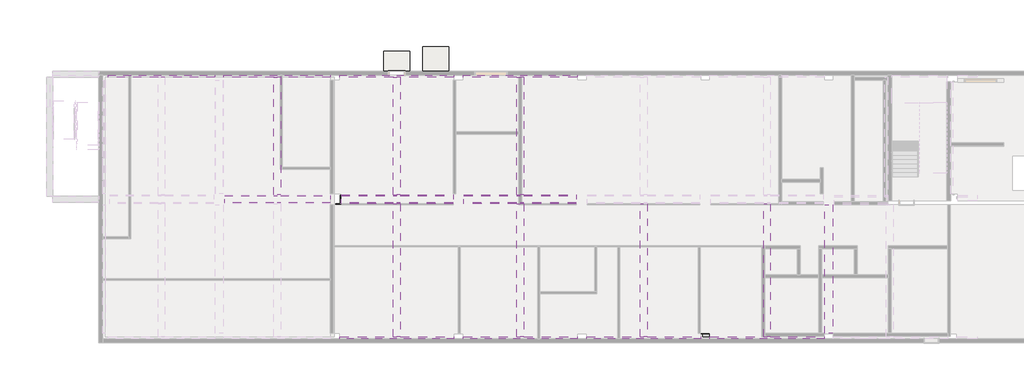
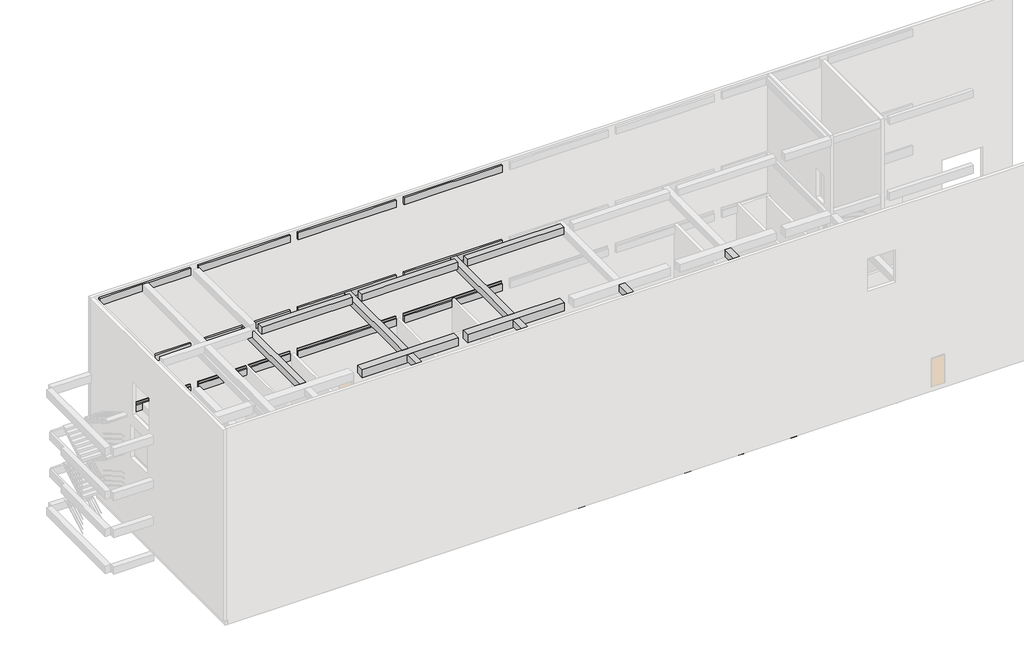
# One storey, part 3 of 5: 54 beams, 2 slabs.
# Revit data of these elements (continued)
# Type "RC Beam_Rectangular : H_SB_AR_S16_UG_B500xH700_1G1"
#   Type Comments = "CV-UG"
#   Type Mark = "1G1"
#   H_Q'ty Cal Type Tag = "SB-Q1"
#   H_WM Code_1 = "A03AF032-00022 |  | M3 | Concrete Work | Superstructure Work | Structural Concrete | Cement Type-1 | 25MPa ≤ F'c (Cylinder Strength) < 30MPa |  |  |  |  | A03AF032-00022 Concrete Work Superstructure Work Structural Concrete  Cement Type-1 25MPa ≤ F'c (Cylinder Strength) < 30MPa      |  F'c (Cylinder Strength) = 24MPa"
#   H_WM Code_2 = "A03AD037-00002 |  | TON | Concrete Work | Substructure Work | Rebar Work | Deformed Bar (Non-Coat.) | 400MPa<Fy≤470MPa |  |  |  |  | A03AD037-00002 Concrete Work Substructure Work Rebar Work Deformed Bar (Non-Coat.)  400MPa<Fy≤470MPa      | ASTM A615 GRADE 60 (Fy=420MPa)"
#   H_WM Code_3 = "A03AF036-00001 |  | M2 | Concrete Work | Superstructure Work | Form Work (1 time in use) | Flat Form | Dressed Lumber, Plywood or Steel Form(Wood Planks are not Allowed) incl. Chamfer |  |  |  | A03AF036-00001 Concrete Work Superstructure Work Form Work (1 time in use) Flat Form     Dressed Lumber, Plywood or Steel Form(Wood Planks are not Allowed) incl. Chamfer   |"
#   중앙부 하부근 = ""
#   중앙부 상부근 = ""
#   중앙부 보조근 = ""
#   중앙부 늑근 = ""
#   외단부 하부근 = ""
#   외단부 상부근 = ""
#   외단부 보조근 = ""
#   외단부 늑근 = ""
#   부호 = "TG2"
#   내단부 하부근 = ""
#   내단부 상부근 = ""
#   내단부 보조근 = ""
#   내단부 늑근 = ""
#   ALL 하부근 = "3-D20"
#   ALL 상부근 = "4-D20"
#   ALL 보조근 = ""
#   ALL 늑근 = "2-D10 @120"
#   H_Rebar ratio = 0.14
#   Width = 500 mm
#   Height = 700 mm
#   Length [instance default] = 1524 mm
#   b = 500 mm
#   h = 700 mm
#   hec_material3 [instance default] = none
#   hec_material2 [instance default] = none
#   hec_material1 [instance default] = none
#   Structural Material [instance default] = none
#   Assembly Code = ""
# Type "RC Beam_Rectangular : H_SB_AR_S16_UG_B450xH700_1B1A"
#   Type Comments = "UG"
#   Type Mark = "1B1A"
#   H_Q'ty Cal Type Tag = "SB-Q1"
#   H_WM Code_1 = "A03AF032-00022 |  | M3 | Concrete Work | Superstructure Work | Structural Concrete | Cement Type-1 | 25MPa ≤ F'c (Cylinder Strength) < 30MPa |  |  |  |  | A03AF032-00022 Concrete Work Superstructure Work Structural Concrete  Cement Type-1 25MPa ≤ F'c (Cylinder Strength) < 30MPa      |  F'c (Cylinder Strength) = 24MPa"
#   H_WM Code_2 = "A03AD037-00002 |  | TON | Concrete Work | Substructure Work | Rebar Work | Deformed Bar (Non-Coat.) | 400MPa<Fy≤470MPa |  |  |  |  | A03AD037-00002 Concrete Work Substructure Work Rebar Work Deformed Bar (Non-Coat.)  400MPa<Fy≤470MPa      | ASTM A615 GRADE 60 (Fy=420MPa)"
#   H_WM Code_3 = "A03AF036-00001 |  | M2 | Concrete Work | Superstructure Work | Form Work (1 time in use) | Flat Form | Dressed Lumber, Plywood or Steel Form(Wood Planks are not Allowed) incl. Chamfer |  |  |  | A03AF036-00001 Concrete Work Superstructure Work Form Work (1 time in use) Flat Form     Dressed Lumber, Plywood or Steel Form(Wood Planks are not Allowed) incl. Chamfer   |"
#   중앙부 하부근 = ""
#   중앙부 상부근 = ""
#   중앙부 보조근 = ""
#   중앙부 늑근 = ""
#   외단부 하부근 = ""
#   외단부 상부근 = ""
#   외단부 보조근 = ""
#   외단부 늑근 = ""
#   부호 = "TG2"
#   내단부 하부근 = ""
#   내단부 상부근 = ""
#   내단부 보조근 = ""
#   내단부 늑근 = ""
#   ALL 하부근 = "3-D20"
#   ALL 상부근 = "4-D20"
#   ALL 보조근 = ""
#   ALL 늑근 = "2-D10 @120"
#   Width = 450 mm
#   Height = 700 mm
#   Length [instance default] = 1524 mm
#   b = 450 mm
#   h = 700 mm
#   hec_material3 [instance default] = none
#   hec_material2 [instance default] = none
#   hec_material1 [instance default] = none
#   Structural Material [instance default] = none
#   Assembly Code = ""
# Type "RC Beam_Rectangular : H_SB_AR_S16_AG_B400xH700_3WG1"
#   Type Comments = "CV-AG"
#   Type Mark = "3WG1"
#   H_Q'ty Cal Type Tag = "SB-Q1"
#   H_WM Code_1 = "A03AF032-00022 |  | M3 | Concrete Work | Superstructure Work | Structural Concrete | Cement Type-1 | 25MPa ≤ F'c (Cylinder Strength) < 30MPa |  |  |  |  | A03AF032-00022 Concrete Work Superstructure Work Structural Concrete  Cement Type-1 25MPa ≤ F'c (Cylinder Strength) < 30MPa      |  F'c (Cylinder Strength) = 24MPa"
#   H_WM Code_2 = "A03AD037-00002 |  | TON | Concrete Work | Substructure Work | Rebar Work | Deformed Bar (Non-Coat.) | 400MPa<Fy≤470MPa |  |  |  |  | A03AD037-00002 Concrete Work Substructure Work Rebar Work Deformed Bar (Non-Coat.)  400MPa<Fy≤470MPa      | ASTM A615 GRADE 60 (Fy=420MPa)"
#   H_WM Code_3 = "A03AF036-00001 |  | M2 | Concrete Work | Superstructure Work | Form Work (1 time in use) | Flat Form | Dressed Lumber, Plywood or Steel Form(Wood Planks are not Allowed) incl. Chamfer |  |  |  | A03AF036-00001 Concrete Work Superstructure Work Form Work (1 time in use) Flat Form     Dressed Lumber, Plywood or Steel Form(Wood Planks are not Allowed) incl. Chamfer   |"
#   중앙부 하부근 = ""
#   중앙부 상부근 = ""
#   중앙부 보조근 = ""
#   중앙부 늑근 = ""
#   외단부 하부근 = ""
#   외단부 상부근 = ""
#   외단부 보조근 = ""
#   외단부 늑근 = ""
#   부호 = "TG2"
#   내단부 하부근 = ""
#   내단부 상부근 = ""
#   내단부 보조근 = ""
#   내단부 늑근 = ""
#   ALL 하부근 = "3-D20"
#   ALL 상부근 = "4-D20"
#   ALL 보조근 = ""
#   ALL 늑근 = "2-D10 @120"
#   H_Rebar ratio = 0.14
#   Width = 400 mm
#   Height = 700 mm
#   Length [instance default] = 1524 mm
#   b = 400 mm
#   h = 700 mm
#   hec_material3 [instance default] = none
#   hec_material2 [instance default] = none
#   hec_material1 [instance default] = none
#   Structural Material [instance default] = none
#   Assembly Code = ""
# Type "RC Beam_Rectangular : H_SB_AR_S16_AG_B600xH800_3G2"
#   Type Comments = "AG"
#   Type Mark = "3G2"
#   H_Q'ty Cal Type Tag = "SB-Q1"
#   H_WM Code_1 = "A03AF032-00022 |  | M3 | Concrete Work | Superstructure Work | Structural Concrete | Cement Type-1 | 25MPa ≤ F'c (Cylinder Strength) < 30MPa |  |  |  |  | A03AF032-00022 Concrete Work Superstructure Work Structural Concrete  Cement Type-1 25MPa ≤ F'c (Cylinder Strength) < 30MPa      |  F'c (Cylinder Strength) = 24MPa"
#   H_WM Code_2 = "A03AD037-00002 |  | TON | Concrete Work | Substructure Work | Rebar Work | Deformed Bar (Non-Coat.) | 400MPa<Fy≤470MPa |  |  |  |  | A03AD037-00002 Concrete Work Substructure Work Rebar Work Deformed Bar (Non-Coat.)  400MPa<Fy≤470MPa      | ASTM A615 GRADE 60 (Fy=420MPa)"
#   H_WM Code_3 = "A03AF036-00001 |  | M2 | Concrete Work | Superstructure Work | Form Work (1 time in use) | Flat Form | Dressed Lumber, Plywood or Steel Form(Wood Planks are not Allowed) incl. Chamfer |  |  |  | A03AF036-00001 Concrete Work Superstructure Work Form Work (1 time in use) Flat Form     Dressed Lumber, Plywood or Steel Form(Wood Planks are not Allowed) incl. Chamfer   |"
#   중앙부 하부근 = ""
#   중앙부 상부근 = ""
#   중앙부 보조근 = ""
#   중앙부 늑근 = ""
#   외단부 하부근 = ""
#   외단부 상부근 = ""
#   외단부 보조근 = ""
#   외단부 늑근 = ""
#   부호 = "TG2"
#   내단부 하부근 = ""
#   내단부 상부근 = ""
#   내단부 보조근 = ""
#   내단부 늑근 = ""
#   ALL 하부근 = "3-D20"
#   ALL 상부근 = "4-D20"
#   ALL 보조근 = ""
#   ALL 늑근 = "2-D10 @120"
#   Width = 600 mm
#   Height = 800 mm
#   Length [instance default] = 1524 mm
#   b = 600 mm
#   h = 800 mm
#   hec_material3 [instance default] = none
#   hec_material2 [instance default] = none
#   hec_material1 [instance default] = none
#   Structural Material [instance default] = none
#   Assembly Code = ""
# Type "RC Beam_Rectangular : H_SB_AR_S16_AG_B4500xH700_3G1"
#   Type Comments = "AG"
#   Type Mark = "3G1"
#   H_Q'ty Cal Type Tag = "SB-Q1"
#   H_WM Code_1 = "A03AF032-00022 |  | M3 | Concrete Work | Superstructure Work | Structural Concrete | Cement Type-1 | 25MPa ≤ F'c (Cylinder Strength) < 30MPa |  |  |  |  | A03AF032-00022 Concrete Work Superstructure Work Structural Concrete  Cement Type-1 25MPa ≤ F'c (Cylinder Strength) < 30MPa      |  F'c (Cylinder Strength) = 24MPa"
#   H_WM Code_2 = "A03AD037-00002 |  | TON | Concrete Work | Substructure Work | Rebar Work | Deformed Bar (Non-Coat.) | 400MPa<Fy≤470MPa |  |  |  |  | A03AD037-00002 Concrete Work Substructure Work Rebar Work Deformed Bar (Non-Coat.)  400MPa<Fy≤470MPa      | ASTM A615 GRADE 60 (Fy=420MPa)"
#   H_WM Code_3 = "A03AF036-00001 |  | M2 | Concrete Work | Superstructure Work | Form Work (1 time in use) | Flat Form | Dressed Lumber, Plywood or Steel Form(Wood Planks are not Allowed) incl. Chamfer |  |  |  | A03AF036-00001 Concrete Work Superstructure Work Form Work (1 time in use) Flat Form     Dressed Lumber, Plywood or Steel Form(Wood Planks are not Allowed) incl. Chamfer   |"
#   중앙부 하부근 = ""
#   중앙부 상부근 = ""
#   중앙부 보조근 = ""
#   중앙부 늑근 = ""
#   외단부 하부근 = ""
#   외단부 상부근 = ""
#   외단부 보조근 = ""
#   외단부 늑근 = ""
#   부호 = "TG2"
#   내단부 하부근 = ""
#   내단부 상부근 = ""
#   내단부 보조근 = ""
#   내단부 늑근 = ""
#   ALL 하부근 = "3-D20"
#   ALL 상부근 = "4-D20"
#   ALL 보조근 = ""
#   ALL 늑근 = "2-D10 @120"
#   Width = 500 mm
#   Height = 700 mm
#   Length [instance default] = 1524 mm
#   b = 500 mm
#   h = 700 mm
#   hec_material3 [instance default] = none
#   hec_material2 [instance default] = none
#   hec_material1 [instance default] = none
#   Structural Material [instance default] = none
#   Assembly Code = ""
# Type "RC Beam_Rectangular : H_SB_AR_S16_AG_B450xH700_3B1"
#   Type Comments = "AG"
#   Type Mark = "3B1"
#   H_Q'ty Cal Type Tag = "SB-Q1"
#   H_WM Code_1 = "A03AF032-00022 |  | M3 | Concrete Work | Superstructure Work | Structural Concrete | Cement Type-1 | 25MPa ≤ F'c (Cylinder Strength) < 30MPa |  |  |  |  | A03AF032-00022 Concrete Work Superstructure Work Structural Concrete  Cement Type-1 25MPa ≤ F'c (Cylinder Strength) < 30MPa      |  F'c (Cylinder Strength) = 24MPa"
#   H_WM Code_2 = "A03AD037-00002 |  | TON | Concrete Work | Substructure Work | Rebar Work | Deformed Bar (Non-Coat.) | 400MPa<Fy≤470MPa |  |  |  |  | A03AD037-00002 Concrete Work Substructure Work Rebar Work Deformed Bar (Non-Coat.)  400MPa<Fy≤470MPa      | ASTM A615 GRADE 60 (Fy=420MPa)"
#   H_WM Code_3 = "A03AF036-00001 |  | M2 | Concrete Work | Superstructure Work | Form Work (1 time in use) | Flat Form | Dressed Lumber, Plywood or Steel Form(Wood Planks are not Allowed) incl. Chamfer |  |  |  | A03AF036-00001 Concrete Work Superstructure Work Form Work (1 time in use) Flat Form     Dressed Lumber, Plywood or Steel Form(Wood Planks are not Allowed) incl. Chamfer   |"
#   중앙부 하부근 = ""
#   중앙부 상부근 = ""
#   중앙부 보조근 = ""
#   중앙부 늑근 = ""
#   외단부 하부근 = ""
#   외단부 상부근 = ""
#   외단부 보조근 = ""
#   외단부 늑근 = ""
#   부호 = "TG2"
#   내단부 하부근 = ""
#   내단부 상부근 = ""
#   내단부 보조근 = ""
#   내단부 늑근 = ""
#   ALL 하부근 = "3-D20"
#   ALL 상부근 = "4-D20"
#   ALL 보조근 = ""
#   ALL 늑근 = "2-D10 @120"
#   Width = 450 mm
#   Height = 700 mm
#   Length [instance default] = 1524 mm
#   b = 450 mm
#   h = 700 mm
#   hec_material3 [instance default] = none
#   hec_material2 [instance default] = none
#   hec_material1 [instance default] = none
#   Structural Material [instance default] = none
#   Assembly Code = ""
# Type "RC Beam_Rectangular : H_SB_AR_S16_AG_B450xH700_3B1A"
#   Type Comments = "AG"
#   Type Mark = "3B1A"
#   H_Q'ty Cal Type Tag = "SB-Q1"
#   H_WM Code_1 = "A03AF032-00022 |  | M3 | Concrete Work | Superstructure Work | Structural Concrete | Cement Type-1 | 25MPa ≤ F'c (Cylinder Strength) < 30MPa |  |  |  |  | A03AF032-00022 Concrete Work Superstructure Work Structural Concrete  Cement Type-1 25MPa ≤ F'c (Cylinder Strength) < 30MPa      |  F'c (Cylinder Strength) = 24MPa"
#   H_WM Code_2 = "A03AD037-00002 |  | TON | Concrete Work | Substructure Work | Rebar Work | Deformed Bar (Non-Coat.) | 400MPa<Fy≤470MPa |  |  |  |  | A03AD037-00002 Concrete Work Substructure Work Rebar Work Deformed Bar (Non-Coat.)  400MPa<Fy≤470MPa      | ASTM A615 GRADE 60 (Fy=420MPa)"
#   H_WM Code_3 = "A03AF036-00001 |  | M2 | Concrete Work | Superstructure Work | Form Work (1 time in use) | Flat Form | Dressed Lumber, Plywood or Steel Form(Wood Planks are not Allowed) incl. Chamfer |  |  |  | A03AF036-00001 Concrete Work Superstructure Work Form Work (1 time in use) Flat Form     Dressed Lumber, Plywood or Steel Form(Wood Planks are not Allowed) incl. Chamfer   |"
#   중앙부 하부근 = ""
#   중앙부 상부근 = ""
#   중앙부 보조근 = ""
#   중앙부 늑근 = ""
#   외단부 하부근 = ""
#   외단부 상부근 = ""
#   외단부 보조근 = ""
#   외단부 늑근 = ""
#   부호 = "TG2"
#   내단부 하부근 = ""
#   내단부 상부근 = ""
#   내단부 보조근 = ""
#   내단부 늑근 = ""
#   ALL 하부근 = "3-D20"
#   ALL 상부근 = "4-D20"
#   ALL 보조근 = ""
#   ALL 늑근 = "2-D10 @120"
#   Width = 450 mm
#   Height = 700 mm
#   Length [instance default] = 1524 mm
#   b = 450 mm
#   h = 700 mm
#   hec_material3 [instance default] = none
#   hec_material2 [instance default] = none
#   hec_material1 [instance default] = none
#   Structural Material [instance default] = none
#   Assembly Code = ""
# Type "RC Beam_Rectangular : H_SB_AR_S16_AG_B400xH700_RWG1"
#   Type Comments = "CV-AG"
#   Type Mark = "RWG1"
#   H_Q'ty Cal Type Tag = "SB-Q1"
#   H_WM Code_1 = "A03AF032-00022 |  | M3 | Concrete Work | Superstructure Work | Structural Concrete | Cement Type-1 | 25MPa ≤ F'c (Cylinder Strength) < 30MPa |  |  |  |  | A03AF032-00022 Concrete Work Superstructure Work Structural Concrete  Cement Type-1 25MPa ≤ F'c (Cylinder Strength) < 30MPa      |  F'c (Cylinder Strength) = 24MPa"
#   H_WM Code_2 = "A03AD037-00002 |  | TON | Concrete Work | Substructure Work | Rebar Work | Deformed Bar (Non-Coat.) | 400MPa<Fy≤470MPa |  |  |  |  | A03AD037-00002 Concrete Work Substructure Work Rebar Work Deformed Bar (Non-Coat.)  400MPa<Fy≤470MPa      | ASTM A615 GRADE 60 (Fy=420MPa)"
#   H_WM Code_3 = "A03AF036-00001 |  | M2 | Concrete Work | Superstructure Work | Form Work (1 time in use) | Flat Form | Dressed Lumber, Plywood or Steel Form(Wood Planks are not Allowed) incl. Chamfer |  |  |  | A03AF036-00001 Concrete Work Superstructure Work Form Work (1 time in use) Flat Form     Dressed Lumber, Plywood or Steel Form(Wood Planks are not Allowed) incl. Chamfer   |"
#   중앙부 하부근 = ""
#   중앙부 상부근 = ""
#   중앙부 보조근 = ""
#   중앙부 늑근 = ""
#   외단부 하부근 = ""
#   외단부 상부근 = ""
#   외단부 보조근 = ""
#   외단부 늑근 = ""
#   부호 = "TG2"
#   내단부 하부근 = ""
#   내단부 상부근 = ""
#   내단부 보조근 = ""
#   내단부 늑근 = ""
#   ALL 하부근 = "3-D20"
#   ALL 상부근 = "4-D20"
#   ALL 보조근 = ""
#   ALL 늑근 = "2-D10 @120"
#   H_Rebar ratio = 0.14
#   Width = 400 mm
#   Height = 700 mm
#   Length [instance default] = 1524 mm
#   b = 400 mm
#   h = 700 mm
#   hec_material3 [instance default] = none
#   hec_material2 [instance default] = none
#   hec_material1 [instance default] = none
#   Structural Material [instance default] = none
#   Assembly Code = ""
# Type "RC Beam_Rectangular : H_SB_AR_S16_AG_B450xH700_RG2"
#   Type Comments = "AG"
#   Type Mark = "RG2"
#   H_Q'ty Cal Type Tag = "SB-Q1"
#   H_WM Code_1 = "A03AF032-00022 |  | M3 | Concrete Work | Superstructure Work | Structural Concrete | Cement Type-1 | 25MPa ≤ F'c (Cylinder Strength) < 30MPa |  |  |  |  | A03AF032-00022 Concrete Work Superstructure Work Structural Concrete  Cement Type-1 25MPa ≤ F'c (Cylinder Strength) < 30MPa      |  F'c (Cylinder Strength) = 24MPa"
#   H_WM Code_2 = "A03AD037-00002 |  | TON | Concrete Work | Substructure Work | Rebar Work | Deformed Bar (Non-Coat.) | 400MPa<Fy≤470MPa |  |  |  |  | A03AD037-00002 Concrete Work Substructure Work Rebar Work Deformed Bar (Non-Coat.)  400MPa<Fy≤470MPa      | ASTM A615 GRADE 60 (Fy=420MPa)"
#   H_WM Code_3 = "A03AF036-00001 |  | M2 | Concrete Work | Superstructure Work | Form Work (1 time in use) | Flat Form | Dressed Lumber, Plywood or Steel Form(Wood Planks are not Allowed) incl. Chamfer |  |  |  | A03AF036-00001 Concrete Work Superstructure Work Form Work (1 time in use) Flat Form     Dressed Lumber, Plywood or Steel Form(Wood Planks are not Allowed) incl. Chamfer   |"
#   중앙부 하부근 = ""
#   중앙부 상부근 = ""
#   중앙부 보조근 = ""
#   중앙부 늑근 = ""
#   외단부 하부근 = ""
#   외단부 상부근 = ""
#   외단부 보조근 = ""
#   외단부 늑근 = ""
#   부호 = "TG2"
#   내단부 하부근 = ""
#   내단부 상부근 = ""
#   내단부 보조근 = ""
#   내단부 늑근 = ""
#   ALL 하부근 = "3-D20"
#   ALL 상부근 = "4-D20"
#   ALL 보조근 = ""
#   ALL 늑근 = "2-D10 @120"
#   Width = 450 mm
#   Height = 700 mm
#   Length [instance default] = 1524 mm
#   b = 450 mm
#   h = 700 mm
#   hec_material3 [instance default] = none
#   hec_material2 [instance default] = none
#   hec_material1 [instance default] = none
#   Structural Material [instance default] = none
#   Assembly Code = ""
# Type "H_SF_AR_B08_Ramp_Ramp2"
#   Type Comments = "CV-AG"
#   Type Mark = "Ramp2"
#   H_Q'ty Cal Type Tag = "SB-Q1A"
#   H_WM Code_1 = "A03AF032-00022 |  | M3 | Concrete Work | Superstructure Work | Structural Concrete | Cement Type-1 | 25MPa ≤ F'c (Cylinder Strength) < 30MPa |  |  |  |  | A03AF032-00022 Concrete Work Superstructure Work Structural Concrete  Cement Type-1 25MPa ≤ F'c (Cylinder Strength) < 30MPa      |  F'c (Cylinder Strength) = 24MPa"
#   H_WM Code_2 = "A03AD037-00002 |  | TON | Concrete Work | Substructure Work | Rebar Work | Deformed Bar (Non-Coat.) | 400MPa<Fy≤470MPa |  |  |  |  | A03AD037-00002 Concrete Work Substructure Work Rebar Work Deformed Bar (Non-Coat.)  400MPa<Fy≤470MPa      | ASTM A615 GRADE 60 (Fy=420MPa)"
#   H_WM Code_3 = "A03AD035-00001 |  | M2 | Concrete Work | Substructure Work | Form Work (3 times in use) | Flat Form | Dressed Lumber, Plywood or Steel Form(Wood Planks are not Allowed) incl. Chamfer |  |  |  | A03AD035-00001 Concrete Work Substructure Work Form Work (3 times in use) Flat Form     Dressed Lumber, Plywood or Steel Form(Wood Planks are not Allowed) incl. Chamfer   | Dressed Lumber, Plywood or Steel Form(Wood Planks are not Allowed) incl. Chamfer"
#   H_WM Code_4 = "A03AH056-00001 |  | M2 | Concrete Work | Concrete Protective Coating (U/G) | Bitumen/Bituminous/Asphalt Coating |  |  | A03AH056-00001 Concrete Work Concrete Protective Coating (U/G) Bitumen/Bituminous/Asphalt Coating         | Bitumen/Bituminous/Asphalt Coating"
#   H_WM Code_5 = "A03AD047-00004 |  | M2 | Concrete Work | Substructure Work | Insulation under Ground Floor | Extruded Polystyrene Insulation Board |  | 100mm≤THK | THK=(  )mm |  | A03AD047-00004 Concrete Work Substructure Work Insulation under Ground Floor Extruded Polystyrene Insulation Board       100mm≤THK | Bitumen/Bituminous/Asphalt Coating"
#   H_WM Code_6 = "A01ZZ001-00012 |  | M3 | Earth Work | - | Excavation | Soil, Mech. |  | Manual Excavation Above GWL |  |  |  | A01ZZ001-00012 Earth Work - Excavation Soil, Mech.      Manual Excavation Above GWL  | Above GWL"
#   H_WM Code_7 = "A01ZZ001-00013 |  | M3 | Earth Work | - | Excavation | Soil, Mech. |  | Manual Excavation Below GWL |  |  |  | A01ZZ001-00013 Earth Work - Excavation Soil, Mech.      Manual Excavation Below GWL  | Below GWL"
#   H_WM Code_8 = "A01ZZ003-00001 |  | M3 | Earth Work | - | Backfill | Re-use, Soil |  |  |  | Compaction=(  )% |  | A01ZZ003-00001 Earth Work - Backfill Re-use, Soil        | Compaction=( 95 )%"
#   H_WM Code_9 = "A01ZZ004-00001 |  | M3 | Earth Work | - | Disposal | Soil |  |  |  | Disposal Distance=Appx. (  )km from Site |  | A01ZZ004-00001 Earth Work - Disposal Soil        | Disposal Distance=Appx. (20 )km from Site"
#   H_WM Code_10 = "A03AH056-00001 |  | M2 | Concrete Work | Concrete Protective Coating (U/G) | Bitumen/Bituminous/Asphalt Coating |  |  | A03AH056-00001 Concrete Work Concrete Protective Coating (U/G) Bitumen/Bituminous/Asphalt Coating         | *기초바닥 Protection 은 Lean에 적용"
#   H_Rebar ratio = 0.1
#   Layers, outside or top first: 0 mm no material (function 100); 200 mm "00_Concrete_Reinf. Conc." (function 1); 0 mm no material (function 100); 0 mm no material (function 100)
# Element 1 (IfcBeam, "RC Beam_Rectangular : H_SB_AR_S16_UG_B600xH800_1G2")
#   Comments = ""
#   hec_material3 = none
#   hec_material2 = none
#   hec_material1 = none
#   Structural Material = 00_Concrete_Reinf. Conc.
#   Phase Created = New Construction
#   Materials on its faces: "00_Concrete_Reinf. Conc."
# Elements 2, 3 (IfcBeam, "RC Beam_Rectangular : H_SB_AR_S16_UG_B450xH700_1B1")
#   Comments = ""
#   hec_material3 = none
#   hec_material2 = none
#   hec_material1 = none
#   Structural Material = 00_Concrete_Reinf. Conc.
#   Phase Created = New Construction
#   Materials on its faces: "00_Concrete_Reinf. Conc."
# Elements 4, 5, 6, 7, 8, 9 (IfcBeam, "RC Beam_Rectangular : H_SB_AR_S16_UG_B500xH700_1G1")
#   Comments = ""
#   hec_material3 = none
#   hec_material2 = none
#   hec_material1 = none
#   Structural Material = 00_Concrete_Reinf. Conc.
#   Phase Created = New Construction
#   Materials on its faces: "00_Concrete_Reinf. Conc."
# Elements 10, 11, 12, 13 (IfcBeam, "RC Beam_Rectangular : H_SB_AR_S16_UG_B450xH700_1B1A")
#   Comments = ""
#   hec_material3 = none
#   hec_material2 = none
#   hec_material1 = none
#   Structural Material = none
#   Phase Created = New Construction
# Elements 14, 15, 16, 17, 18, 19, 20, 21, 25, 26, 27, 28, 29, 30, 31, 32 (IfcBeam, "RC Beam_Rectangular : H_SB_AR_S16_AG_B400xH700_3WG1")
#   Comments = ""
#   hec_material3 = none
#   hec_material2 = none
#   hec_material1 = none
#   Structural Material = 00_Concrete_Reinf. Conc.
#   Phase Created = New Construction
#   Materials on its faces: "00_Concrete_Reinf. Conc."
# Elements 22, 23, 33, 34 (IfcBeam, "RC Beam_Rectangular : H_SB_AR_S16_AG_B600xH800_3G2")
#   Comments = ""
#   hec_material3 = none
#   hec_material2 = none
#   hec_material1 = none
#   Structural Material = none
#   Phase Created = New Construction
# Element 24 (IfcBeam, "RC Beam_Rectangular : H_SB_AR_S16_AG_B4500xH700_3G1")
#   Comments = ""
#   hec_material3 = none
#   hec_material2 = none
#   hec_material1 = none
#   Structural Material = none
#   Phase Created = New Construction
# Elements 35, 36, 37 (IfcBeam, "RC Beam_Rectangular : H_SB_AR_S16_AG_B450xH700_3B1")
#   Comments = ""
#   hec_material3 = none
#   hec_material2 = none
#   hec_material1 = none
#   Structural Material = none
#   Phase Created = New Construction
# Elements 38, 39, 40, 41 (IfcBeam, "RC Beam_Rectangular : H_SB_AR_S16_AG_B450xH700_3B1A")
#   Comments = ""
#   hec_material3 = none
#   hec_material2 = none
#   hec_material1 = none
#   Structural Material = none
#   Phase Created = New Construction
# Elements 42, 43, 44, 45, 46, 47, 48, 49 (IfcBeam, "RC Beam_Rectangular : H_SB_AR_S16_AG_B400xH700_RWG1")
#   Comments = ""
#   hec_material3 = none
#   hec_material2 = none
#   hec_material1 = none
#   Structural Material = 00_Concrete_Reinf. Conc.
#   Phase Created = New Construction
#   Materials on its faces: "00_Concrete_Reinf. Conc."
# Elements 50, 51, 52 (IfcBeam, "RC Beam_Rectangular : H_SB_AR_S16_AG_B450xH700_RG2")
#   Comments = ""
#   hec_material3 = none
#   hec_material2 = none
#   hec_material1 = none
#   Structural Material = none
#   Phase Created = New Construction
# Element 53 (IfcBeam, "RC Beam_Rectangular : H_SB_AR_S16_UG_B600xH800_1G2")
#   IfcGUID = "0DKOmQSjf1KgvfYSs63FG0"
#   Comments = ""
#   Phase Created = New Construction
#   Materials on its faces: "00_Concrete_Reinf. Conc."
# Element 54 (IfcBeam, "RC Beam_Rectangular : H_SB_AR_S16_UG_B600xH800_1G2")
#   IfcGUID = "0DKOmQSjf1KgvfYSs63FHI"
#   Comments = ""
#   Phase Created = New Construction
#   Materials on its faces: "00_Concrete_Reinf. Conc."
# Elements 55, 56 (IfcSlab, "H_SF_AR_B08_Ramp_Ramp2")
#   Comments = ""
#   built-in parameter 1001955 = 3.14159 (stored number, unit not read)
#   Height Offset From Level = 0 mm
#   built-in parameter 1001954 = 1
#   Phase Created = New Construction
# Materials
#   "00_Concrete_Reinf. Conc.": class "Concrete", colour RGB 176 176 176, transparency 0, Description = "Reinf. Conc.", Cost = 0, Image = Concrete.Cast-In-Place.Flat.Polished.Grey.jpg
# Room at (48881.519, 2598.242) mm, phase "New Construction", upper level "TOC", upper offset 9000 mm, lower offset 0 mm
#   Comments = ""
#   Number = "121"
#   Name = "TOILET (M)"
#   H_Floor Finish Style Name = "Non-Slip Unglazed Ceramic Tile"
#   H_Floor Base Material = "Concrete Slab / Screed / Liquid Waterproofing"
#   H_Wall-Base Material-1 = "Masonry Wall"
#   H_Wall-Base Material-2 = ""
#   H_Wall-Base Material-3 = ""
#   H_Floor-Base Material-1 = "Concrete Slab"
#   H_Floor-Base Material-2 = ""
#   H_Floor-Base Material-3 = "Screed"
#   H_Floor-Base Material-4 = "Liquid Waterproofing"
#   H_Floor-Base Material-5 = "Ceramic Tile"
#   H_Floor Finish-1 = "Ceramic Tile"
#   H_Floor Finish-2 = ""
#   H_Floor Finish Remark = ""
#   H_Wall Finish Style Name = "Glazed Ceramic Tile (≤C.H+100) / No Paint (>C.H+100)"
#   H_Wall Base Material = "Masonry Wall"
#   H_Wall-Base Material-4 = "No Waterproofing"
#   H_Wall-Base Material-5 = "Glazed Ceramic Tile"
#   H_Wall Finish-1 = "Glazed Ceramic Tile"
#   H_Wall Finish-2 = ""
#   H_Wall Finish Remark = "Below Suspended Ceiling\nGlazed Ceramic Tile(≤C.H+100) / No Paint (>C.H+100)"
#   H_Ceiling Finish Style Name = "Suspended Gypsum Plaster Board Ceiling (M-Bar)"
#   H_Ceiling Base Material = "Concrete Slab / Fair Faced Concrete"
#   H_Ceiling-Base Material-1 = "(Concrete Slab)"
#   H_Ceiling-Base Material-2 = "(Fair Faced Concrete)"
#   H_Ceiling-Base Material-3 = ""
#   H_Ceiling-Base Material-4 = ""
#   H_Ceiling-Base Material-5 = "Gypsum Plaster Board Ceiling System"
#   H_Ceiling Finish-1 = "Gypsum Plaster Board Ceiling System"
#   H_Ceiling Finish-2 = ""
#   H_Ceiling Finish Remark = ""
#   H_Room W = 3800 mm
#   H_Room L = 5600 mm
#   H_Room H or CH = 9000 mm
#   Floor Finish Style No = none
#   Wall Finish Style No = W32D
#   Ceiling Finish Style No = C92
# Room at (40583.851, 3309.471) mm, phase "New Construction", upper level "TOC", upper offset 9000 mm, lower offset 0 mm
#   Comments = ""
#   Number = "117"
#   Name = "PARTNER'S ROOM"
#   H_Floor Finish Style Name = "Vinyl Tile"
#   H_Floor Base Material = "Concrete Slab / Steel Trowel Finish"
#   H_Wall-Base Material-1 = "Masonry Wall"
#   H_Skirt Finish Style Name = "Coved Vinyl Tile"
#   H_Wall-Base Material-2 = ""
#   H_Wall-Base Material-3 = "Plastering"
#   H_Floor-Base Material-1 = "Concrete Slab"
#   H_Floor-Base Material-2 = "Steel Trowel Finish"
#   H_Floor-Base Material-3 = ""
#   H_Floor-Base Material-4 = ""
#   H_Floor-Base Material-5 = "Vinyl Tile"
#   H_Floor Finish-1 = "Vinyl Tile"
#   H_Floor Finish-2 = ""
#   H_Floor Finish Remark = ""
#   H_Skirt Base Material = "Same as Wall"
#   H_Skirt-Base Material-1 = ""
#   H_Skirt-Base Material-2 = ""
#   H_Skirt-Base Material-3 = ""
#   H_Skirt-Base Material-4 = ""
#   H_Skirt-Base Material-5 = ""
#   H_Skirt Finish-1 = "Vinyl Tile"
#   H_Skirt Finish-2 = ""
#   H_Skirt Finish Remark = "Vinyl Tile = PVC Tile (polyvinyl chloride)"
#   H_Wall Finish Style Name = "Water Emulsion Paint"
#   H_Wall Base Material = "Masonry Wall / Cement Plaster"
#   H_Wall-Base Material-4 = ""
#   H_Wall-Base Material-5 = ""
#   H_Wall Finish-1 = ""
#   H_Wall Finish-2 = ""
#   H_Wall Finish Remark = ""
#   H_Ceiling Finish Style Name = "Suspended Acoustic Tiled Ceiling (M-Bar)"
#   H_Ceiling Base Material = "Concrete Slab / Fair Faced Concrete"
#   H_Ceiling-Base Material-1 = "(Concrete Slab)"
#   H_Ceiling-Base Material-2 = "(Fair Faced Concrete)"
#   H_Ceiling-Base Material-3 = ""
#   H_Ceiling-Base Material-4 = ""
#   H_Ceiling-Base Material-5 = "Acoustic Tiled Ceiling System (M-Bar)"
#   H_Ceiling Finish-1 = "Acoustic Tiled Ceiling System (M-Bar)"
#   H_Ceiling Finish-2 = ""
#   H_Ceiling Finish Remark = ""
#   H_Room W = 3700 mm
#   H_Room L = 3700 mm
#   H_Room H or CH = 9000 mm
#   Floor Finish Style No = none
#   Skirt Finish Style No = none
#   Wall Finish Style No = W02B
#   Ceiling Finish Style No = C95A
# Room at (25580.312, 3648.151) mm, phase "New Construction", upper level "TOC", upper offset 9000 mm, lower offset 0 mm
#   Comments = ""
#   Number = "115"
#   Name = "REST ROOM"
#   H_Floor Finish Style Name = "Vinyl Tile"
#   H_Floor Base Material = "Concrete Slab / Steel Trowel Finish"
#   H_Wall-Base Material-1 = "Masonry Wall"
#   H_Skirt Finish Style Name = "Coved Vinyl Tile"
#   H_Wall-Base Material-2 = ""
#   H_Wall-Base Material-3 = "Plastering"
#   H_Floor-Base Material-1 = "Concrete Slab"
#   H_Floor-Base Material-2 = "Steel Trowel Finish"
#   H_Floor-Base Material-3 = ""
#   H_Floor-Base Material-4 = ""
#   H_Floor-Base Material-5 = "Vinyl Tile"
#   H_Floor Finish-1 = "Vinyl Tile"
#   H_Floor Finish-2 = ""
#   H_Floor Finish Remark = ""
#   H_Skirt Base Material = "Same as Wall"
#   H_Skirt-Base Material-1 = ""
#   H_Skirt-Base Material-2 = ""
#   H_Skirt-Base Material-3 = ""
#   H_Skirt-Base Material-4 = ""
#   H_Skirt-Base Material-5 = ""
#   H_Skirt Finish-1 = "Vinyl Tile"
#   H_Skirt Finish-2 = ""
#   H_Skirt Finish Remark = "Vinyl Tile = PVC Tile (polyvinyl chloride)"
#   H_Wall Finish Style Name = "Water Emulsion Paint"
#   H_Wall Base Material = "Masonry Wall / Cement Plaster"
#   H_Wall-Base Material-4 = ""
#   H_Wall-Base Material-5 = ""
#   H_Wall Finish-1 = ""
#   H_Wall Finish-2 = ""
#   H_Wall Finish Remark = ""
#   H_Ceiling Finish Style Name = "Suspended Gypsum Plaster Board Ceiling (M-Bar)"
#   H_Ceiling Base Material = "Concrete Slab / Fair Faced Concrete"
#   H_Ceiling-Base Material-1 = "(Concrete Slab)"
#   H_Ceiling-Base Material-2 = "(Fair Faced Concrete)"
#   H_Ceiling-Base Material-3 = ""
#   H_Ceiling-Base Material-4 = ""
#   H_Ceiling-Base Material-5 = "Gypsum Plaster Board Ceiling System"
#   H_Ceiling Finish-1 = "Gypsum Plaster Board Ceiling System"
#   H_Ceiling Finish-2 = ""
#   H_Ceiling Finish Remark = ""
#   H_Room W = 3700 mm
#   H_Room L = 3000 mm
#   H_Room H or CH = 9000 mm
#   Floor Finish Style No = none
#   Skirt Finish Style No = none
#   Wall Finish Style No = W02B
#   Ceiling Finish Style No = C92
# Room at (6490.87, 11650.959) mm, phase "New Construction", upper level "TOC", upper offset 9000 mm, lower offset 0 mm
#   Comments = ""
#   Number = "101"
#   Name = "CENTRAL CONTROL ROOM"
#   H_Floor Finish Style Name = "Anti-Dust Epoxy Paint / Anti-Static Vinyl Tile on Raised Floor"
#   H_Floor Base Material = "Concrete Slab / Steel Trowel Finish"
#   H_Wall-Base Material-1 = "Masonry Wall"
#   H_Skirt Finish Style Name = "Coved Vinyl Tile"
#   H_Wall-Base Material-2 = ""
#   H_Wall-Base Material-3 = "Plastering"
#   H_Floor-Base Material-1 = "Concrete Slab"
#   H_Floor-Base Material-2 = "Steel Trowel Finish"
#   H_Floor-Base Material-3 = ""
#   H_Floor-Base Material-4 = ""
#   H_Floor-Base Material-5 = "Raised Floor_Anti-Static Vinyl Tile"
#   H_Floor Finish-1 = "Anti-Dust Paint"
#   H_Floor Finish-2 = "Raised Floor_Anti-Static Vinyl Tile"
#   H_Floor Finish Remark = "600x600, H=1000"
#   H_Skirt Base Material = "Same as Wall"
#   H_Skirt-Base Material-1 = ""
#   H_Skirt-Base Material-2 = ""
#   H_Skirt-Base Material-3 = ""
#   H_Skirt-Base Material-4 = ""
#   H_Skirt-Base Material-5 = ""
#   H_Skirt Finish-1 = "Vinyl Tile"
#   H_Skirt Finish-2 = ""
#   H_Skirt Finish Remark = "Vinyl Tile = PVC Tile (polyvinyl chloride)"
#   H_Wall Finish Style Name = "Water Emulsion Paint"
#   H_Wall Base Material = "Masonry Wall / Cement Plaster"
#   H_Wall-Base Material-4 = ""
#   H_Wall-Base Material-5 = ""
#   H_Wall Finish-1 = ""
#   H_Wall Finish-2 = ""
#   H_Wall Finish Remark = ""
#   H_Ceiling Finish Style Name = "Suspended Acoustic Tiled Ceiling (M-Bar)"
#   H_Ceiling Base Material = "Concrete Slab / Fair Faced Concrete"
#   H_Ceiling-Base Material-1 = "(Concrete Slab)"
#   H_Ceiling-Base Material-2 = "(Fair Faced Concrete)"
#   H_Ceiling-Base Material-3 = ""
#   H_Ceiling-Base Material-4 = ""
#   H_Ceiling-Base Material-5 = "Acoustic Tiled Ceiling System (M-Bar)"
#   H_Ceiling Finish-1 = "Acoustic Tiled Ceiling System (M-Bar)"
#   H_Ceiling Finish-2 = ""
#   H_Ceiling Finish Remark = ""
#   H_Room W = 14900 mm
#   H_Room L = 13300 mm
#   H_Room H or CH = 9000 mm
#   Floor Finish Style No = none
#   Skirt Finish Style No = none
#   Wall Finish Style No = W02B
#   Ceiling Finish Style No = C95A
# Room at (904.971, 12877.131) mm, phase "New Construction", upper level "TOC", upper offset 9000 mm, lower offset 0 mm
#   Comments = ""
#   Number = "127"
#   Name = "NONE"
#   H_Floor Finish Style Name = "Anti-Dust Epoxy Paint / Anti-Static Vinyl Tile on Raised Floor"
#   H_Floor Base Material = "Concrete Slab / Steel Trowel Finish"
#   H_Wall-Base Material-1 = "Masonry Wall"
#   H_Skirt Finish Style Name = "Coved Vinyl Tile"
#   H_Wall-Base Material-2 = ""
#   H_Wall-Base Material-3 = "Plastering"
#   H_Floor-Base Material-1 = "Concrete Slab"
#   H_Floor-Base Material-2 = "Steel Trowel Finish"
#   H_Floor-Base Material-3 = ""
#   H_Floor-Base Material-4 = ""
#   H_Floor-Base Material-5 = "Raised Floor_Anti-Static Vinyl Tile"
#   H_Floor Finish-1 = "Anti-Dust Paint"
#   H_Floor Finish-2 = "Raised Floor_Anti-Static Vinyl Tile"
#   H_Floor Finish Remark = "600x600, H=1000"
#   H_Skirt Base Material = "Same as Wall"
#   H_Skirt-Base Material-1 = ""
#   H_Skirt-Base Material-2 = ""
#   H_Skirt-Base Material-3 = ""
#   H_Skirt-Base Material-4 = ""
#   H_Skirt-Base Material-5 = ""
#   H_Skirt Finish-1 = "Vinyl Tile"
#   H_Skirt Finish-2 = ""
#   H_Skirt Finish Remark = "Vinyl Tile = PVC Tile (polyvinyl chloride)"
#   H_Wall Finish Style Name = "Water Emulsion Paint"
#   H_Wall Base Material = "Masonry Wall / Cement Plaster"
#   H_Wall-Base Material-4 = ""
#   H_Wall-Base Material-5 = ""
#   H_Wall Finish-1 = ""
#   H_Wall Finish-2 = ""
#   H_Wall Finish Remark = ""
#   H_Ceiling Finish Style Name = "Suspended Acoustic Tiled Ceiling (M-Bar)"
#   H_Ceiling Base Material = "Concrete Slab / Fair Faced Concrete"
#   H_Ceiling-Base Material-1 = "(Concrete Slab)"
#   H_Ceiling-Base Material-2 = "(Fair Faced Concrete)"
#   H_Ceiling-Base Material-3 = ""
#   H_Ceiling-Base Material-4 = ""
#   H_Ceiling-Base Material-5 = "Acoustic Tiled Ceiling System (M-Bar)"
#   H_Ceiling Finish-1 = "Acoustic Tiled Ceiling System (M-Bar)"
#   H_Ceiling Finish-2 = ""
#   H_Ceiling Finish Remark = ""
#   H_Room W = 700 mm
#   H_Room L = 700 mm
#   H_Room H or CH = 9000 mm
#   Floor Finish Style No = none
#   Skirt Finish Style No = none
#   Wall Finish Style No = W02B
#   Ceiling Finish Style No = C95A
# Room at (13098.579, 14171.425) mm, phase "New Construction", upper level "TOC", upper offset 9000 mm, lower offset 0 mm
#   Comments = ""
#   Number = "102"
#   Name = "MEETING ROOM"
#   H_Floor Finish Style Name = "Anti-Dust Epoxy Paint / Anti-Static Vinyl Tile on Raised Floor"
#   H_Floor Base Material = "Concrete Slab / Steel Trowel Finish"
#   H_Wall-Base Material-1 = "Masonry Wall"
#   H_Skirt Finish Style Name = "Coved Vinyl Tile"
#   H_Wall-Base Material-2 = ""
#   H_Wall-Base Material-3 = "Plastering"
#   H_Floor-Base Material-1 = "Concrete Slab"
#   H_Floor-Base Material-2 = "Steel Trowel Finish"
#   H_Floor-Base Material-3 = ""
#   H_Floor-Base Material-4 = ""
#   H_Floor-Base Material-5 = "Raised Floor_Anti-Static Vinyl Tile"
#   H_Floor Finish-1 = "Anti-Dust Paint"
#   H_Floor Finish-2 = "Raised Floor_Anti-Static Vinyl Tile"
#   H_Floor Finish Remark = "600x600, H=1000"
#   H_Skirt Base Material = "Same as Wall"
#   H_Skirt-Base Material-1 = ""
#   H_Skirt-Base Material-2 = ""
#   H_Skirt-Base Material-3 = ""
#   H_Skirt-Base Material-4 = ""
#   H_Skirt-Base Material-5 = ""
#   H_Skirt Finish-1 = "Vinyl Tile"
#   H_Skirt Finish-2 = ""
#   H_Skirt Finish Remark = "Vinyl Tile = PVC Tile (polyvinyl chloride)"
#   H_Wall Finish Style Name = "Water Emulsion Paint"
#   H_Wall Base Material = "Masonry Wall / Cement Plaster"
#   H_Wall-Base Material-4 = ""
#   H_Wall-Base Material-5 = ""
#   H_Wall Finish-1 = ""
#   H_Wall Finish-2 = ""
#   H_Wall Finish Remark = ""
#   H_Ceiling Finish Style Name = "Suspended Moisture Resistant Tiled Ceiling (T-Bar)"
#   H_Ceiling Base Material = "Concrete Slab / Fair Faced Concrete"
#   H_Ceiling-Base Material-1 = "(Concrete Slab)"
#   H_Ceiling-Base Material-2 = "(Fair Faced Concrete)"
#   H_Ceiling-Base Material-3 = ""
#   H_Ceiling-Base Material-4 = ""
#   H_Ceiling-Base Material-5 = "Moisture Resistant Tiled Ceiling System (T-Bar)"
#   H_Ceiling Finish-1 = "Moisture Resistant Tiled Ceiling System (T-Bar)"
#   H_Ceiling Finish-2 = ""
#   H_Ceiling Finish Remark = "600x600\nT bar"
#   H_Room W = 1800 mm
#   H_Room L = 10600 mm
#   H_Room H or CH = 9000 mm
#   Floor Finish Style No = none
#   Skirt Finish Style No = none
#   Wall Finish Style No = W02B
#   Ceiling Finish Style No = C96B
# Room at (6967.715, 2863.387) mm, phase "New Construction", upper level "TOC", upper offset 9000 mm, lower offset 0 mm
#   Comments = ""
#   Number = "103"
#   Name = "ENGINEERING ROOM"
#   H_Floor Finish Style Name = "Anti-Dust Epoxy Paint / Anti-Static Vinyl Tile on Raised Floor"
#   H_Floor Base Material = "Concrete Slab / Steel Trowel Finish"
#   H_Wall-Base Material-1 = "Masonry Wall"
#   H_Skirt Finish Style Name = "Coved Vinyl Tile"
#   H_Wall-Base Material-2 = ""
#   H_Wall-Base Material-3 = "Plastering"
#   H_Floor-Base Material-1 = "Concrete Slab"
#   H_Floor-Base Material-2 = "Steel Trowel Finish"
#   H_Floor-Base Material-3 = ""
#   H_Floor-Base Material-4 = ""
#   H_Floor-Base Material-5 = "Raised Floor_Anti-Static Vinyl Tile"
#   H_Floor Finish-1 = "Anti-Dust Paint"
#   H_Floor Finish-2 = "Raised Floor_Anti-Static Vinyl Tile"
#   H_Floor Finish Remark = "600x600, H=1000"
#   H_Skirt Base Material = "Same as Wall"
#   H_Skirt-Base Material-1 = ""
#   H_Skirt-Base Material-2 = ""
#   H_Skirt-Base Material-3 = ""
#   H_Skirt-Base Material-4 = ""
#   H_Skirt-Base Material-5 = ""
#   H_Skirt Finish-1 = "Vinyl Tile"
#   H_Skirt Finish-2 = ""
#   H_Skirt Finish Remark = "Vinyl Tile = PVC Tile (polyvinyl chloride)"
#   H_Wall Finish Style Name = "Water Emulsion Paint"
#   H_Wall Base Material = "Masonry Wall / Cement Plaster"
#   H_Wall-Base Material-4 = ""
#   H_Wall-Base Material-5 = ""
#   H_Wall Finish-1 = ""
#   H_Wall Finish-2 = ""
#   H_Wall Finish Remark = ""
#   H_Ceiling Finish Style Name = "Suspended Acoustic Tiled Ceiling (M-Bar)"
#   H_Ceiling Base Material = "Concrete Slab / Fair Faced Concrete"
#   H_Ceiling-Base Material-1 = "(Concrete Slab)"
#   H_Ceiling-Base Material-2 = "(Fair Faced Concrete)"
#   H_Ceiling-Base Material-3 = ""
#   H_Ceiling-Base Material-4 = ""
#   H_Ceiling-Base Material-5 = "Acoustic Tiled Ceiling System (M-Bar)"
#   H_Ceiling Finish-1 = "Acoustic Tiled Ceiling System (M-Bar)"
#   H_Ceiling Finish-2 = ""
#   H_Ceiling Finish Remark = ""
#   H_Room W = 3200 mm
#   H_Room L = 6100 mm
#   H_Room H or CH = 9000 mm
#   Floor Finish Style No = none
#   Skirt Finish Style No = none
#   Wall Finish Style No = W02B
#   Ceiling Finish Style No = C95A
# Room at (18684.477, 14171.425) mm, phase "New Construction", upper level "TOC", upper offset 9000 mm, lower offset 0 mm
#   Comments = ""
#   Number = "104"
#   Name = "CANTEEN"
#   H_Floor Finish Style Name = "Vinyl Tile"
#   H_Floor Base Material = "Concrete Slab / Screed"
#   H_Wall-Base Material-1 = "Masonry Wall"
#   H_Skirt Finish Style Name = "Coved Vinyl Tile"
#   H_Wall-Base Material-2 = ""
#   H_Wall-Base Material-3 = "Plastering"
#   H_Floor-Base Material-1 = "Concrete Slab"
#   H_Floor-Base Material-2 = ""
#   H_Floor-Base Material-3 = "Screed"
#   H_Floor-Base Material-4 = ""
#   H_Floor-Base Material-5 = "Vinyl Tile"
#   H_Floor Finish-1 = "Vinyl Tile"
#   H_Floor Finish-2 = ""
#   H_Floor Finish Remark = ""
#   H_Skirt Base Material = "Same as Wall"
#   H_Skirt-Base Material-1 = ""
#   H_Skirt-Base Material-2 = ""
#   H_Skirt-Base Material-3 = ""
#   H_Skirt-Base Material-4 = ""
#   H_Skirt-Base Material-5 = ""
#   H_Skirt Finish-1 = "Vinyl Tile"
#   H_Skirt Finish-2 = ""
#   H_Skirt Finish Remark = "Vinyl Tile = PVC Tile (polyvinyl chloride)"
#   H_Wall Finish Style Name = "Water Emulsion Paint"
#   H_Wall Base Material = "Masonry Wall / Cement Plaster"
#   H_Wall-Base Material-4 = ""
#   H_Wall-Base Material-5 = ""
#   H_Wall Finish-1 = ""
#   H_Wall Finish-2 = ""
#   H_Wall Finish Remark = ""
#   H_Ceiling Finish Style Name = "Suspended Gypsum Plaster Board Ceiling (M-Bar)"
#   H_Ceiling Base Material = "Concrete Slab / Fair Faced Concrete"
#   H_Ceiling-Base Material-1 = "(Concrete Slab)"
#   H_Ceiling-Base Material-2 = "(Fair Faced Concrete)"
#   H_Ceiling-Base Material-3 = ""
#   H_Ceiling-Base Material-4 = ""
#   H_Ceiling-Base Material-5 = "Gypsum Plaster Board Ceiling System"
#   H_Ceiling Finish-1 = "Gypsum Plaster Board Ceiling System"
#   H_Ceiling Finish-2 = ""
#   H_Ceiling Finish Remark = ""
#   H_Room W = 14900 mm
#   H_Room L = 3900 mm
#   H_Room H or CH = 9000 mm
#   Floor Finish Style No = none
#   Skirt Finish Style No = none
#   Wall Finish Style No = W02B
#   Ceiling Finish Style No = C92
# Room at (24679.1, 15942.564) mm, phase "New Construction", upper level "TOC", upper offset 9000 mm, lower offset 0 mm
#   Comments = ""
#   Number = "105"
#   Name = "AIR LOCK"
#   H_Floor Finish Style Name = "Non-Slip Unglazed Ceramic Tile"
#   H_Floor Base Material = "Concrete Slab / Steel Trowel Finish"
#   H_Wall-Base Material-1 = "Masonry Wall"
#   H_Skirt Finish Style Name = "Coved Vinyl Tile"
#   H_Wall-Base Material-2 = ""
#   H_Wall-Base Material-3 = "Plastering"
#   H_Floor-Base Material-1 = "Concrete Slab"
#   H_Floor-Base Material-2 = "Steel Trowel Finish"
#   H_Floor-Base Material-3 = ""
#   H_Floor-Base Material-4 = ""
#   H_Floor-Base Material-5 = "Ceramic Tile"
#   H_Floor Finish-1 = "Ceramic Tile"
#   H_Floor Finish-2 = ""
#   H_Floor Finish Remark = "*WM : Bonding용 Mortar은 Tile에 포함\n*Slope 용 Screed만 별도 구분 (Concrete 바닥 단차 발생하는 경우 Only)"
#   H_Skirt Base Material = "Same as Wall"
#   H_Skirt-Base Material-1 = ""
#   H_Skirt-Base Material-2 = ""
#   H_Skirt-Base Material-3 = ""
#   H_Skirt-Base Material-4 = ""
#   H_Skirt-Base Material-5 = ""
#   H_Skirt Finish-1 = "Vinyl Tile"
#   H_Skirt Finish-2 = ""
#   H_Skirt Finish Remark = "Vinyl Tile = PVC Tile (polyvinyl chloride)"
#   H_Wall Finish Style Name = "Water Emulsion Paint"
#   H_Wall Base Material = "Masonry Wall / Cement Plaster"
#   H_Wall-Base Material-4 = ""
#   H_Wall-Base Material-5 = ""
#   H_Wall Finish-1 = ""
#   H_Wall Finish-2 = ""
#   H_Wall Finish Remark = ""
#   H_Ceiling Finish Style Name = "Suspended Gypsum Plaster Board Ceiling (M-Bar)"
#   H_Ceiling Base Material = "Concrete Slab / Fair Faced Concrete"
#   H_Ceiling-Base Material-1 = "(Concrete Slab)"
#   H_Ceiling-Base Material-2 = "(Fair Faced Concrete)"
#   H_Ceiling-Base Material-3 = ""
#   H_Ceiling-Base Material-4 = ""
#   H_Ceiling-Base Material-5 = "Gypsum Plaster Board Ceiling System"
#   H_Ceiling Finish-1 = "Gypsum Plaster Board Ceiling System"
#   H_Ceiling Finish-2 = ""
#   H_Ceiling Finish Remark = ""
#   H_Room W = 7900 mm
#   H_Room L = 8400 mm
#   H_Room H or CH = 9000 mm
#   Floor Finish Style No = none
#   Skirt Finish Style No = none
#   Wall Finish Style No = W02B
#   Ceiling Finish Style No = C92
# Room at (24679.1, 11446.597) mm, phase "New Construction", upper level "TOC", upper offset 9000 mm, lower offset 0 mm
#   Comments = ""
#   Number = "106"
#   Name = "LOBBY"
#   H_Floor Finish Style Name = "Vinyl Tile"
#   H_Floor Base Material = "Concrete Slab / Steel Trowel Finish"
#   H_Wall-Base Material-1 = "Masonry Wall"
#   H_Skirt Finish Style Name = "Coved Vinyl Tile"
#   H_Wall-Base Material-2 = ""
#   H_Wall-Base Material-3 = "Plastering"
#   H_Floor-Base Material-1 = "Concrete Slab"
#   H_Floor-Base Material-2 = "Steel Trowel Finish"
#   H_Floor-Base Material-3 = ""
#   H_Floor-Base Material-4 = ""
#   H_Floor-Base Material-5 = "Vinyl Tile"
#   H_Floor Finish-1 = "Vinyl Tile"
#   H_Floor Finish-2 = ""
#   H_Floor Finish Remark = ""
#   H_Skirt Base Material = "Same as Wall"
#   H_Skirt-Base Material-1 = ""
#   H_Skirt-Base Material-2 = ""
#   H_Skirt-Base Material-3 = ""
#   H_Skirt-Base Material-4 = ""
#   H_Skirt-Base Material-5 = ""
#   H_Skirt Finish-1 = "Vinyl Tile"
#   H_Skirt Finish-2 = ""
#   H_Skirt Finish Remark = "Vinyl Tile = PVC Tile (polyvinyl chloride)"
#   H_Wall Finish Style Name = "Water Emulsion Paint"
#   H_Wall Base Material = "Masonry Wall / Cement Plaster"
#   H_Wall-Base Material-4 = ""
#   H_Wall-Base Material-5 = ""
#   H_Wall Finish-1 = ""
#   H_Wall Finish-2 = ""
#   H_Wall Finish Remark = ""
#   H_Ceiling Finish Style Name = "Suspended Gypsum Plaster Board Ceiling (M-Bar)"
#   H_Ceiling Base Material = "Concrete Slab / Fair Faced Concrete"
#   H_Ceiling-Base Material-1 = "(Concrete Slab)"
#   H_Ceiling-Base Material-2 = "(Fair Faced Concrete)"
#   H_Ceiling-Base Material-3 = ""
#   H_Ceiling-Base Material-4 = ""
#   H_Ceiling-Base Material-5 = "Gypsum Plaster Board Ceiling System"
#   H_Ceiling Finish-1 = "Gypsum Plaster Board Ceiling System"
#   H_Ceiling Finish-2 = ""
#   H_Ceiling Finish Remark = ""
#   H_Room W = 4200 mm
#   H_Room L = 3800 mm
#   H_Room H or CH = 9000 mm
#   Floor Finish Style No = none
#   Skirt Finish Style No = none
#   Wall Finish Style No = W02B
#   Ceiling Finish Style No = C92
# Room at (34859.74, 12931.628) mm, phase "New Construction", upper level "TOC", upper offset 9000 mm, lower offset 0 mm
#   Comments = ""
#   Number = "107"
#   Name = "OFFICE ROOM"
#   H_Floor Finish Style Name = "Vinyl Tile"
#   H_Floor Base Material = "Concrete Slab / Steel Trowel Finish"
#   H_Wall-Base Material-1 = "Masonry Wall"
#   H_Skirt Finish Style Name = "Coved Vinyl Tile"
#   H_Wall-Base Material-2 = ""
#   H_Wall-Base Material-3 = "Plastering"
#   H_Floor-Base Material-1 = "Concrete Slab"
#   H_Floor-Base Material-2 = "Steel Trowel Finish"
#   H_Floor-Base Material-3 = ""
#   H_Floor-Base Material-4 = ""
#   H_Floor-Base Material-5 = "Vinyl Tile"
#   H_Floor Finish-1 = "Vinyl Tile"
#   H_Floor Finish-2 = ""
#   H_Floor Finish Remark = ""
#   H_Skirt Base Material = "Same as Wall"
#   H_Skirt-Base Material-1 = ""
#   H_Skirt-Base Material-2 = ""
#   H_Skirt-Base Material-3 = ""
#   H_Skirt-Base Material-4 = ""
#   H_Skirt-Base Material-5 = ""
#   H_Skirt Finish-1 = "Vinyl Tile"
#   H_Skirt Finish-2 = ""
#   H_Skirt Finish Remark = "Vinyl Tile = PVC Tile (polyvinyl chloride)"
#   H_Wall Finish Style Name = "Water Emulsion Paint"
#   H_Wall Base Material = "Masonry Wall / Cement Plaster"
#   H_Wall-Base Material-4 = ""
#   H_Wall-Base Material-5 = ""
#   H_Wall Finish-1 = ""
#   H_Wall Finish-2 = ""
#   H_Wall Finish Remark = ""
#   H_Ceiling Finish Style Name = "Suspended Acoustic Tiled Ceiling (T-Bar)"
#   H_Ceiling Base Material = "Concrete Slab / Fair Faced Concrete"
#   H_Ceiling-Base Material-1 = "(Concrete Slab)"
#   H_Ceiling-Base Material-2 = "(Fair Faced Concrete)"
#   H_Ceiling-Base Material-3 = ""
#   H_Ceiling-Base Material-4 = ""
#   H_Ceiling-Base Material-5 = "Acoustic Tiled Ceiling System (T-Bar)"
#   H_Ceiling Finish-1 = "Acoustic Tiled Ceiling System (T-Bar)"
#   H_Ceiling Finish-2 = ""
#   H_Ceiling Finish Remark = "600x600\nT Bar"
#   H_Room W = 4200 mm
#   H_Room L = 4600 mm
#   H_Room H or CH = 9000 mm
#   Floor Finish Style No = none
#   Skirt Finish Style No = none
#   Wall Finish Style No = W02B
#   Ceiling Finish Style No = C95B
# Room at (45849.496, 13314.591) mm, phase "New Construction", upper level "TOC", upper offset 9000 mm, lower offset 0 mm
#   Comments = ""
#   Number = "108"
#   Name = "LOCKER ROOM"
#   H_Floor Finish Style Name = "Vinyl Tile"
#   H_Floor Base Material = "Concrete Slab / Steel Trowel Finish"
#   H_Wall-Base Material-1 = "Masonry Wall"
#   H_Skirt Finish Style Name = "Coved Vinyl Tile"
#   H_Wall-Base Material-2 = ""
#   H_Wall-Base Material-3 = "Plastering"
#   H_Floor-Base Material-1 = "Concrete Slab"
#   H_Floor-Base Material-2 = "Steel Trowel Finish"
#   H_Floor-Base Material-3 = ""
#   H_Floor-Base Material-4 = ""
#   H_Floor-Base Material-5 = "Vinyl Tile"
#   H_Floor Finish-1 = "Vinyl Tile"
#   H_Floor Finish-2 = ""
#   H_Floor Finish Remark = ""
#   H_Skirt Base Material = "Same as Wall"
#   H_Skirt-Base Material-1 = ""
#   H_Skirt-Base Material-2 = ""
#   H_Skirt-Base Material-3 = ""
#   H_Skirt-Base Material-4 = ""
#   H_Skirt-Base Material-5 = ""
#   H_Skirt Finish-1 = "Vinyl Tile"
#   H_Skirt Finish-2 = ""
#   H_Skirt Finish Remark = "Vinyl Tile = PVC Tile (polyvinyl chloride)"
#   H_Wall Finish Style Name = "Water Emulsion Paint"
#   H_Wall Base Material = "Masonry Wall / Cement Plaster"
#   H_Wall-Base Material-4 = ""
#   H_Wall-Base Material-5 = ""
#   H_Wall Finish-1 = ""
#   H_Wall Finish-2 = ""
#   H_Wall Finish Remark = ""
#   H_Ceiling Finish Style Name = "Suspended Gypsum Plaster Board Ceiling (M-Bar)"
#   H_Ceiling Base Material = "Concrete Slab / Fair Faced Concrete"
#   H_Ceiling-Base Material-1 = "(Concrete Slab)"
#   H_Ceiling-Base Material-2 = "(Fair Faced Concrete)"
#   H_Ceiling-Base Material-3 = ""
#   H_Ceiling-Base Material-4 = ""
#   H_Ceiling-Base Material-5 = "Gypsum Plaster Board Ceiling System"
#   H_Ceiling Finish-1 = "Gypsum Plaster Board Ceiling System"
#   H_Ceiling Finish-2 = ""
#   H_Ceiling Finish Remark = ""
#   H_Room W = 16800 mm
#   H_Room L = 8400 mm
#   H_Room H or CH = 9000 mm
#   Floor Finish Style No = none
#   Skirt Finish Style No = none
#   Wall Finish Style No = W02B
#   Ceiling Finish Style No = C92
# Room at (45344.344, 10064.78) mm, phase "New Construction", upper level "TOC", upper offset 9000 mm, lower offset 0 mm
#   Comments = ""
#   Number = "126"
#   Name = "LOCKER ENTRANCE"
#   H_Floor Finish Style Name = "Non-Slip Epoxy Paint"
#   H_Floor Base Material = "Concrete Slab / Steel Trowel Finish"
#   H_Wall-Base Material-1 = "Masonry Wall"
#   H_Skirt Finish Style Name = "Coved Vinyl Tile"
#   H_Wall-Base Material-2 = ""
#   H_Wall-Base Material-3 = "Plastering"
#   H_Floor-Base Material-1 = "Concrete Slab"
#   H_Floor-Base Material-2 = "Steel Trowel Finish"
#   H_Floor-Base Material-3 = ""
#   H_Floor-Base Material-4 = ""
#   H_Floor-Base Material-5 = ""
#   H_Floor Finish-1 = "Epoxy Paint"
#   H_Floor Finish-2 = ""
#   H_Floor Finish Remark = "*WM 기준 확인 필요 Epoxy Paint \n(용제형, 0.1mm 이하) : epoxy resin + polyamine hardener(경화제)"
#   H_Skirt Base Material = "Same as Wall"
#   H_Skirt-Base Material-1 = ""
#   H_Skirt-Base Material-2 = ""
#   H_Skirt-Base Material-3 = ""
#   H_Skirt-Base Material-4 = ""
#   H_Skirt-Base Material-5 = ""
#   H_Skirt Finish-1 = "Vinyl Tile"
#   H_Skirt Finish-2 = ""
#   H_Skirt Finish Remark = "Vinyl Tile = PVC Tile (polyvinyl chloride)"
#   H_Wall Finish Style Name = "Water Emulsion Paint"
#   H_Wall Base Material = "Masonry Wall / Cement Plaster"
#   H_Wall-Base Material-4 = ""
#   H_Wall-Base Material-5 = ""
#   H_Wall Finish-1 = ""
#   H_Wall Finish-2 = ""
#   H_Wall Finish Remark = ""
#   H_Ceiling Finish Style Name = "Suspended Gypsum Plaster Board Ceiling (M-Bar)"
#   H_Ceiling Base Material = "Concrete Slab / Fair Faced Concrete"
#   H_Ceiling-Base Material-1 = "(Concrete Slab)"
#   H_Ceiling-Base Material-2 = "(Fair Faced Concrete)"
#   H_Ceiling-Base Material-3 = ""
#   H_Ceiling-Base Material-4 = ""
#   H_Ceiling-Base Material-5 = "Gypsum Plaster Board Ceiling System"
#   H_Ceiling Finish-1 = "Gypsum Plaster Board Ceiling System"
#   H_Ceiling Finish-2 = ""
#   H_Ceiling Finish Remark = ""
#   H_Room W = 4700 mm
#   H_Room L = 8400 mm
#   H_Room H or CH = 9000 mm
#   Floor Finish Style No = none
#   Skirt Finish Style No = none
#   Wall Finish Style No = W02B
#   Ceiling Finish Style No = C92
# Room at (49621.297, 12708.408) mm, phase "New Construction", upper level "TOC", upper offset 9000 mm, lower offset 0 mm
#   Comments = ""
#   Number = "109"
#   Name = "SHOWER ROOM"
#   H_Floor Finish Style Name = "Non-Slip Unglazed Ceramic Tile"
#   H_Floor Base Material = "Concrete Slab / Screed / Liquid Waterproof Membrane"
#   H_Wall-Base Material-1 = "Masonry Wall"
#   H_Skirt Finish Style Name = ""
